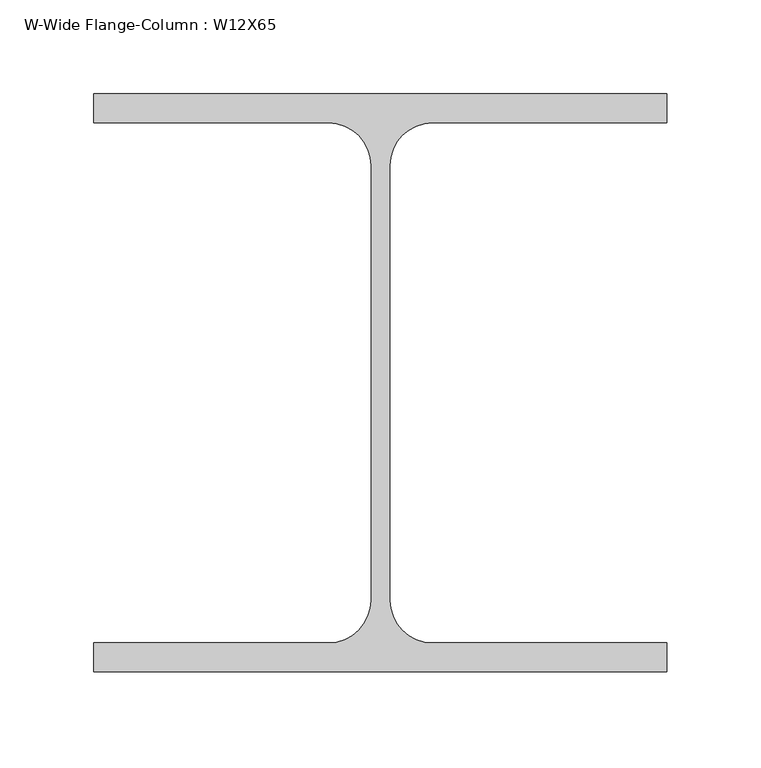
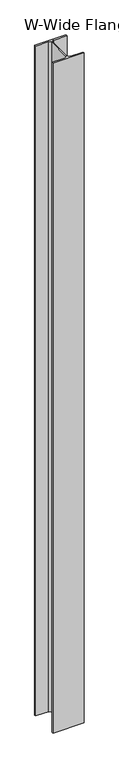
"""IFC4 building model written with IfcOpenShell, lengths in millimetres: column geometry, W-Wide Flange-Column : W12X65."""

from ifc_helpers import new_model, si_unit, point, frame, frame_2d, origin, place, context, project, spatial, polyline, circle_curve, trimmed, segment, composite_curve, outline, extrude, source, transform, mapped, element, save


def w_wide_flange_column_w12x65_f705fd89(model_context):
    return source(origin(), model_context, "Body", "SweptSolid", [
        extrude(outline(composite_curve([segment(polyline([(152.4, 153.67), (152.4, 138.303), (27.686, 138.303)]), True, "CONTINUOUS"), segment(trimmed(circle_curve(frame_2d((27.686, 115.57)), 22.733), [point((27.686, 138.303))], [point((4.953, 115.57))], True, "CARTESIAN"), True, "CONTINUOUS"), segment(polyline([(4.953, 115.57), (4.953, -115.57)]), True, "CONTINUOUS"), segment(trimmed(circle_curve(frame_2d((27.686, -115.57)), 22.733), [point((4.953, -115.57))], [point((27.686, -138.303))], True, "CARTESIAN"), True, "CONTINUOUS"), segment(polyline([(27.686, -138.303), (152.4, -138.303), (152.4, -153.67), (-152.4, -153.67), (-152.4, -138.303), (-27.686, -138.303)]), True, "CONTINUOUS"), segment(trimmed(circle_curve(frame_2d((-27.686, -115.57)), 22.733), [point((-27.686, -138.303))], [point((-4.953, -115.57))], True, "CARTESIAN"), True, "CONTINUOUS"), segment(polyline([(-4.953, -115.57), (-4.953, 115.57)]), True, "CONTINUOUS"), segment(trimmed(circle_curve(frame_2d((-27.686, 115.57)), 22.733), [point((-4.953, 115.57))], [point((-27.686, 138.303))], True, "CARTESIAN"), True, "CONTINUOUS"), segment(polyline([(-27.686, 138.303), (-152.4, 138.303), (-152.4, 153.67), (152.4, 153.67)]), True, "CONTINUOUS")], self_intersect=False)), frame((0.0, 0.0, 16408.4), z_axis=(0.0, 0.0, 1.0), x_axis=(1.0, 0.0, 0.0)), (0.0, 0.0, 1.0), 6908.8),
    ])


if __name__ == "__main__":
    model = new_model("IFC4")
    model_context = context("Model", 3, world=origin())
    ifc_project = project(units=[si_unit("LENGTHUNIT", "METRE", prefix="MILLI")], contexts=[model_context])
    site = spatial("IfcSite", under=ifc_project)
    building = spatial("IfcBuilding", under=site)
    placement = place(None, origin())
    w_wide_flange_column_w12x65_shape = w_wide_flange_column_w12x65_f705fd89(model_context)
    element("IfcColumn", 1, ObjectType="W-Wide Flange-Column : W12X65", at=placement, inside=building, context=model_context, shape_type="MappedRepresentation", body=[
        mapped(w_wide_flange_column_w12x65_shape, transform((0.0, 0.0, 0.0), x_axis=(1.0, 0.0, 0.0), y_axis=(0.0, 1.0, 0.0), z_axis=(0.0, 0.0, 1.0))),
    ])
    save(model, "model.ifc")

# Revit data of these elements
# Type "W-Wide Flange-Column : W12X65"
#   Assembly Code = "B10"
#   W = 65
#   bf = 1' - 0"
#   d = 1' - 0.1"
#   k = 0' - 1 1/2"
#   kr = 0' - 0.895"
#   tf = 0' - 0.605"
#   tw = 0' - 0.39"
#   A = 0.132639 SF
#   Structural Material [instance default] = Steel ASTM A992
# Element 1 (IfcColumn, "W-Wide Flange-Column : W12X65")
#   Materials on its faces: "Steel ASTM A992"
# Materials
#   "Steel ASTM A992": class "Metal", colour RGB 199 199 199, transparency 0, Description = "Structural steel 50ksi", Cost = 0
